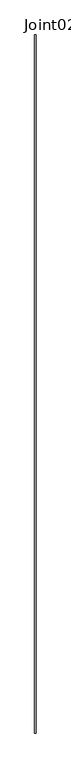
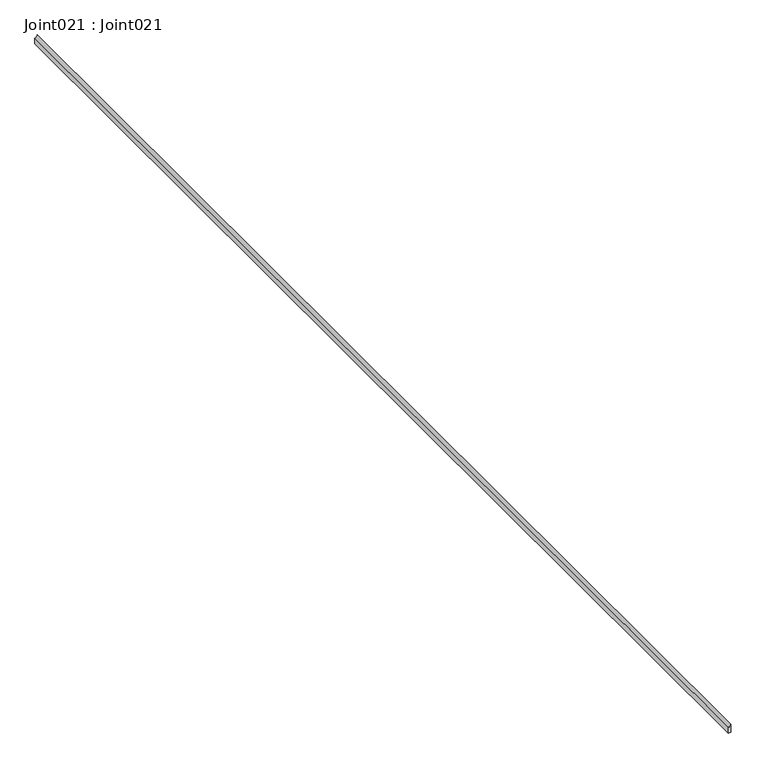
"""IFC4 building model written with IfcOpenShell, lengths in millimetres: proxy geometry, Joint021 : Joint021."""

from ifc_helpers import new_model, si_unit, point, frame, frame_2d, origin, place, context, project, spatial, polyline, circle_curve, trimmed, segment, composite_curve, outline, extrude, source, transform, mapped, element, save


def joint021_joint021_faef97b8(model_context):
    return source(origin(), model_context, "Body", "SweptSolid", [
        extrude(outline(composite_curve([segment(polyline([(42048.0898437, -1094.2821045), (42061.9378947, -1094.2821045)]), True, "CONTINUOUS"), segment(trimmed(circle_curve(frame_2d((42064.2729825, -1100.4790565)), 6.6222994), [point((42061.9378947, -1094.2821045))], [point((42057.9535, -1098.4994125))], True, "CARTESIAN"), True, "CONTINUOUS"), segment(polyline([(42057.9535, -1098.4994125), (42048.0898437, -1098.4994125)]), True, "CONTINUOUS"), segment(trimmed(circle_curve(frame_2d((42040.1796875, -1096.3907585)), 8.1863908), [point((42048.0898437, -1098.4994125))], [point((42048.0898437, -1094.2821045))], True, "CARTESIAN"), True, "CONTINUOUS")], self_intersect=False)), frame((0.0, -1052.8906574, 0.0), z_axis=(0.0, 1.0, 0.0), x_axis=(0.0, 0.0, 1.0)), (0.0, 0.0, 1.0), 2000.0),
    ])


if __name__ == "__main__":
    model = new_model("IFC4")
    model_context = context("Model", 3, world=origin())
    ifc_project = project(units=[si_unit("LENGTHUNIT", "METRE", prefix="MILLI")], contexts=[model_context])
    site = spatial("IfcSite", under=ifc_project)
    building = spatial("IfcBuilding", under=site)
    placement = place(None, origin())
    joint021_joint021_shape = joint021_joint021_faef97b8(model_context)
    element("IfcBuildingElementProxy", 1, Name="Joint021 : Joint021", ObjectType="Joint021 : Joint021", at=placement, inside=building, context=model_context, shape_type="MappedRepresentation", body=[
        mapped(joint021_joint021_shape, transform((0.0, 0.0, 0.0), x_axis=(1.0, 0.0, 0.0), y_axis=(0.0, 1.0, 0.0), z_axis=(0.0, 0.0, 1.0))),
    ])
    save(model, "model.ifc")

# Revit data of these elements
# Type "Joint021 : Joint021"
#   NameOverride = "Joint021"
# Element 1 (IfcBuildingElementProxy, "Joint021 : Joint021")
#   Materials on its faces: "SEALANT JOINT"
# Materials
#   "SEALANT JOINT": class "Unassigned", colour RGB 142 225 148, transparency 0
